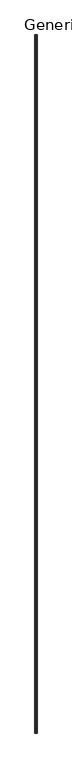
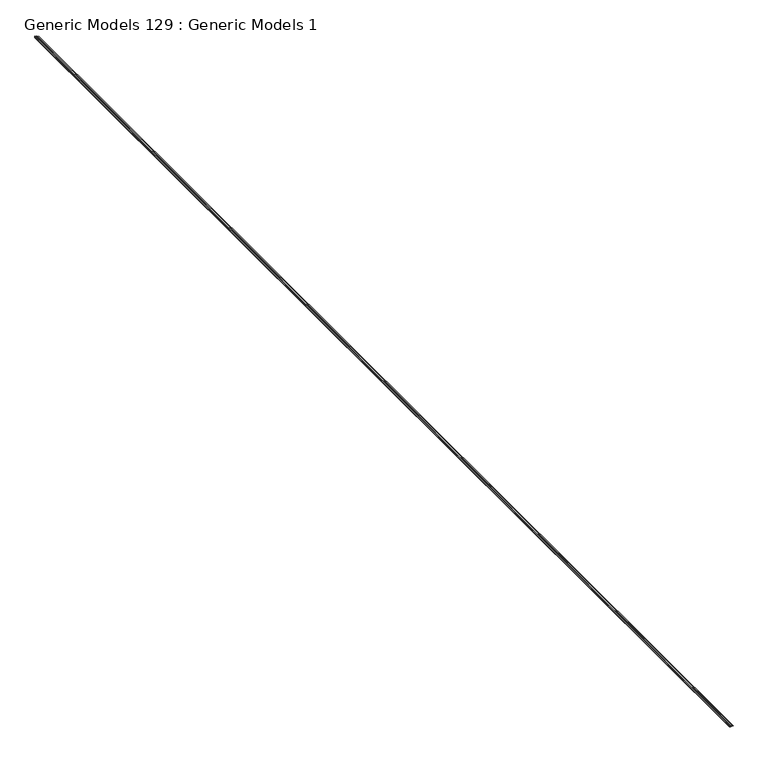
"""IFC4 building model written with IfcOpenShell, lengths in millimetres: proxy geometry, Generic Models 129 : Generic Models 1."""

from ifc_helpers import new_model, si_unit, origin, place, context, project, spatial, faceted_brep, source, transform, mapped, element, save


def generic_models_129_generic_models_1_1b6d92f6(model_context):
    return source(origin(), model_context, "Body", "Brep", [
        faceted_brep([(7074.9963704, 11981.8769662, 126304.421), (7094.6813704, 11981.8769662, 126304.421), (7094.6813704, 11981.8769662, 126315.851), (7109.9213704, 11981.8769662, 126315.851), (7109.9213704, 11981.8769662, 126304.421), (7132.3645544, 11981.8769662, 126304.421), (7132.3645544, 11981.8769662, 126303.151), (7108.6513704, 11981.8769662, 126303.151), (7108.6513704, 11981.8769662, 126314.581), (7095.9513704, 11981.8769662, 126314.581), (7095.9513704, 11981.8769662, 126303.151), (7073.7263704, 11981.8769662, 126303.151), (7073.7263704, 11981.8769662, 126307.9008), (7074.5852113, 11981.8769662, 126307.9008), (7074.5852113, 11981.8769662, 126326.9453787), (7075.8552113, 11981.8769662, 126326.9453787), (7075.8552113, 11981.8769662, 126306.6308), (7074.9963704, 11981.8769662, 126306.6308), (7074.9963704, -7068.1230338, 126304.421), (7074.9963704, -7068.1230338, 126306.6308), (7075.8552113, -7068.1230338, 126306.6308), (7075.8552113, -7068.1230338, 126326.9453787), (7074.5852113, -7068.1230338, 126326.9453787), (7074.5852113, -7068.1230338, 126307.9008), (7073.7263704, -7068.1230338, 126307.9008), (7073.7263704, -7068.1230338, 126303.151), (7095.9513704, -7068.1230338, 126303.151), (7095.9513704, -7068.1230338, 126314.581), (7108.6513704, -7068.1230338, 126314.581), (7108.6513704, -7068.1230338, 126303.151), (7132.3645544, -7068.1230338, 126303.151), (7132.3645544, -7068.1230338, 126304.421), (7109.9213704, -7068.1230338, 126304.421), (7109.9213704, -7068.1230338, 126315.851), (7094.6813704, -7068.1230338, 126315.851), (7094.6813704, -7068.1230338, 126304.421), (7074.9963704, 11778.6769662, 126306.6308), (7074.9963704, -6864.9230338, 126306.6308), (7074.9963704, -6864.9230338, 126304.421), (7074.9963704, 11778.6769662, 126304.421), (7075.8552113, 11778.6769662, 126306.6308), (7075.8552113, -6864.9230338, 126306.6308), (7075.8552113, 11778.6769662, 126326.9453787), (7075.8552113, -6864.9230338, 126326.9453787), (7074.5852113, 11778.6769662, 126326.9453787), (7074.5852113, -6864.9230338, 126326.9453787), (7074.5852113, 11778.6769662, 126307.9008), (7074.5852113, -6864.9230338, 126307.9008), (7073.7263704, 11778.6769662, 126307.9008), (7073.7263704, -6864.9230338, 126307.9008)], [[[0, 1, 2, 3, 4, 5, 6, 7, 8, 9, 10, 11, 12, 13, 14, 15, 16, 17]], [[18, 19, 20, 21, 22, 23, 24, 25, 26, 27, 28, 29, 30, 31, 32, 33, 34, 35]], [[0, 17, 36, 37, 19, 18, 38, 39]], [[17, 16, 40, 41, 20, 19, 37, 36]], [[16, 15, 42, 43, 21, 20, 41, 40]], [[15, 14, 44, 45, 22, 21, 43, 42]], [[14, 13, 46, 47, 23, 22, 45, 44]], [[13, 12, 48, 49, 24, 23, 47, 46]], [[12, 11, 25, 24, 49, 48]], [[11, 10, 26, 25]], [[10, 9, 27, 26]], [[9, 8, 28, 27]], [[8, 7, 29, 28]], [[7, 6, 30, 29]], [[6, 5, 31, 30]], [[5, 4, 32, 31]], [[4, 3, 33, 32]], [[3, 2, 34, 33]], [[2, 1, 35, 34]], [[1, 0, 39, 38, 18, 35]]]),
    ])


if __name__ == "__main__":
    model = new_model("IFC4")
    model_context = context("Model", 3, world=origin())
    ifc_project = project(units=[si_unit("LENGTHUNIT", "METRE", prefix="MILLI")], contexts=[model_context])
    site = spatial("IfcSite", under=ifc_project)
    building = spatial("IfcBuilding", under=site)
    placement = place(None, origin())
    generic_models_129_generic_models_1_shape = generic_models_129_generic_models_1_1b6d92f6(model_context)
    element("IfcBuildingElementProxy", 1, Name="Generic Models 129 : Generic Models 1", ObjectType="Generic Models 129 : Generic Models 1", at=placement, inside=building, context=model_context, shape_type="MappedRepresentation", body=[
        mapped(generic_models_129_generic_models_1_shape, transform((0.0, 0.0, 0.0), x_axis=(1.0, 0.0, 0.0), y_axis=(0.0, 1.0, 0.0), z_axis=(0.0, 0.0, 1.0))),
    ])
    save(model, "model.ifc")

# Revit data of these elements
# Element 1 (IfcBuildingElementProxy, "Generic Models 129 : Generic Models 1")
#   Materials on its faces: "_16 GA. COPPER SOFFIT DRIP SCREED"
# Materials
#   "_16 GA. COPPER SOFFIT DRIP SCREED": class "Generic", colour RGB 253 192 103, transparency 0, Cost = 0
